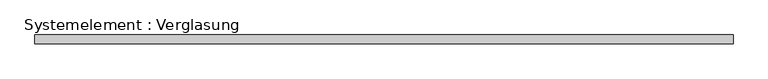
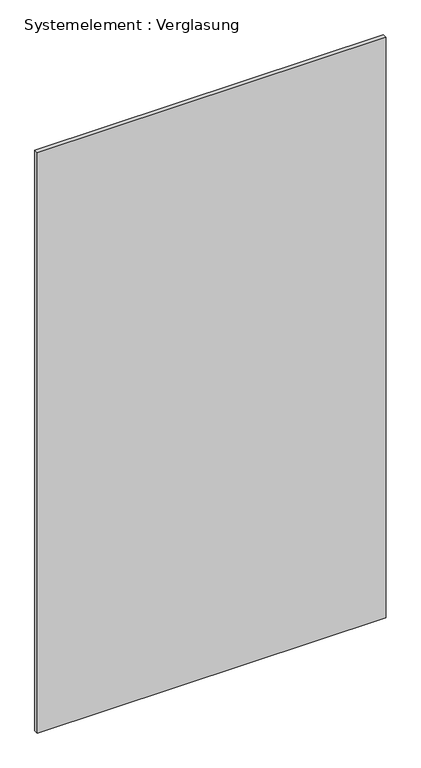
"""IFC4 building model written with IfcOpenShell, lengths in millimetres: plate geometry, Systemelement : Verglasung."""

from ifc_helpers import new_model, si_unit, origin, origin_with_axes, place, context, project, spatial, polyline, outline, extrude, source, transform, mapped, element, save


def systemelement_verglasung_28e5fb00(model_context):
    return source(origin(), model_context, "Body", "SweptSolid", [
        extrude(outline(polyline([(1205.0000002, -15.0), (-1205.0000002, -15.0), (-1205.0000002, 15.0), (1205.0000002, 15.0), (1205.0000002, -15.0)])), origin_with_axes(), (0.0, 0.0, 1.0), 4236.6788019),
    ])


if __name__ == "__main__":
    model = new_model("IFC4")
    model_context = context("Model", 3, world=origin())
    ifc_project = project(units=[si_unit("LENGTHUNIT", "METRE", prefix="MILLI")], contexts=[model_context])
    site = spatial("IfcSite", under=ifc_project)
    building = spatial("IfcBuilding", under=site)
    placement = place(None, origin())
    systemelement_verglasung_shape = systemelement_verglasung_28e5fb00(model_context)
    element("IfcPlate", 1, ObjectType="Systemelement : Verglasung", at=placement, inside=building, context=model_context, shape_type="MappedRepresentation", body=[
        mapped(systemelement_verglasung_shape, transform((0.0, 0.0, 0.0), x_axis=(1.0, 0.0, 0.0), y_axis=(0.0, 1.0, 0.0), z_axis=(0.0, 0.0, 1.0))),
    ])
    save(model, "model.ifc")

# Revit data of these elements
# Type "Systemelement : Verglasung"
#   Construction Type Id = "GSP4R"
#   Analytic Construction = "1/8 Zoll Pilkington-Verglasung einfach"
#   Visual Light Transmittance = 0.9
#   Solar Heat Gain Coefficient = 0.86
#   Heat Transfer Coefficient (U) = 6.7069 W/(m²·K)
# Element 1 (IfcPlate, "Systemelement : Verglasung")
#   Materials on its faces: "Glas"
# Materials
#   "Glas": class "Glas", colour RGB 0 0 255, transparency 0.75, Comments = "Render-Darstellung nicht aktualisiert ", Cost = 0
